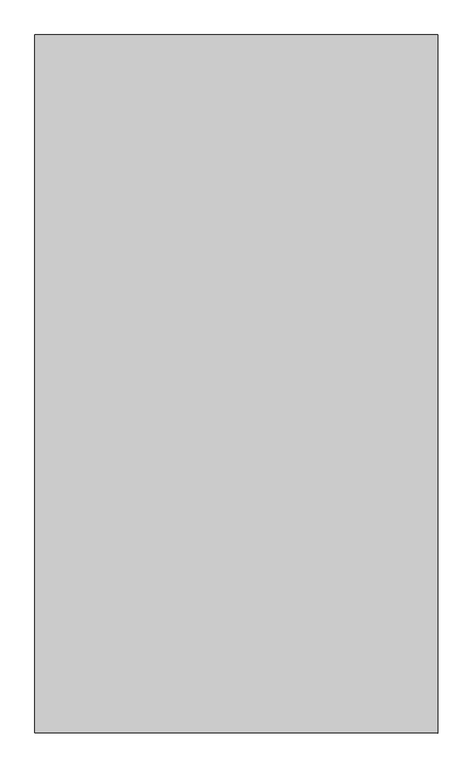
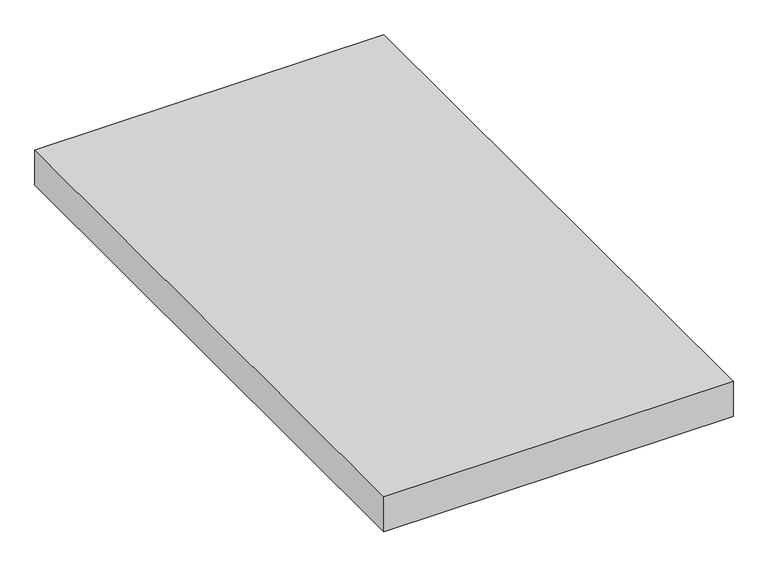
"""IFC4 building model written with IfcOpenShell, lengths in millimetres: proxy geometry, Deckendurchbruch."""

from ifc_helpers import new_model, si_unit, origin, origin_with_axes, place, context, project, spatial, polyline, outline, extrude, source, transform, mapped, element, save


def generic_models_d49041cc(model_context):
    return source(origin(), model_context, "Body", "SweptSolid", [
        extrude(outline(polyline([(0.0, 4420.0), (2550.0, 4420.0), (2550.0, 0.0), (1.23e-05, 1.9161128), (0.0, 4420.0)])), origin_with_axes(), (0.0, 0.0, 1.0), 270.0),
    ])


if __name__ == "__main__":
    model = new_model("IFC4")
    model_context = context("Model", 3, world=origin())
    ifc_project = project(units=[si_unit("LENGTHUNIT", "METRE", prefix="MILLI")], contexts=[model_context])
    site = spatial("IfcSite", under=ifc_project)
    building = spatial("IfcBuilding", under=site)
    placement = place(None, origin())
    generic_models_shape = generic_models_d49041cc(model_context)
    element("IfcBuildingElementProxy", 1, Name="Deckendurchbruch", ObjectType="Deckendurchbruch", at=placement, inside=building, context=model_context, shape_type="MappedRepresentation", body=[
        mapped(generic_models_shape, transform((0.0, 0.0, 0.0), x_axis=(1.0, 0.0, 0.0), y_axis=(0.0, 1.0, 0.0), z_axis=(0.0, 0.0, 1.0))),
    ])
    save(model, "model.ifc")

# Revit data of these elements
# Element 1 (IfcBuildingElementProxy, "Deckendurchbruch")
#   Materials on its faces: "IfcOpeningElement"
# Materials
#   "IfcOpeningElement": class "Unassigned", colour RGB 255 165 0, transparency 0.75
